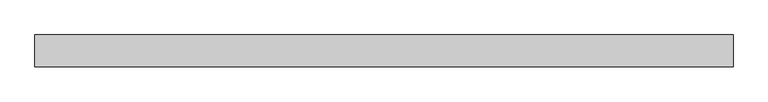
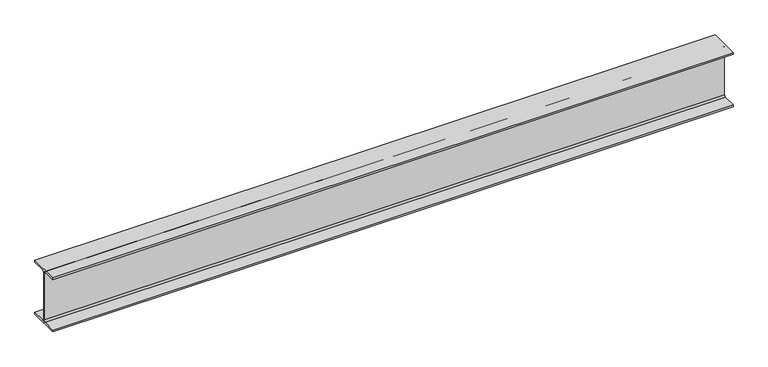
"""IFC4 building model written with IfcOpenShell, lengths in millimetres: beam geometry, Old_Steel Beam_H-KSD3502 : H_SB_ASB_H-250×125x6x9."""

from ifc_helpers import new_model, si_unit, point, frame, frame_2d, origin, place, context, project, spatial, polyline, circle_curve, trimmed, segment, composite_curve, outline, extrude, source, transform, mapped, element, save


def beam_e590c642(model_context):
    return source(origin(), model_context, "Body", "SweptSolid", [
        extrude(outline(composite_curve([segment(polyline([(82.5, -141.5), (82.5, -151.7), (-82.5, -151.7), (-82.5, -141.5), (-11.9, -141.5)]), True, "CONTINUOUS"), segment(trimmed(circle_curve(frame_2d((-11.9, -132.6)), 8.9), [point((-11.9, -141.5))], [point((-3.0, -132.6))], True, "CARTESIAN"), True, "CONTINUOUS"), segment(polyline([(-3.0, -132.6), (-3.0, 132.6)]), True, "CONTINUOUS"), segment(trimmed(circle_curve(frame_2d((-11.9, 132.6)), 8.9), [point((-3.0, 132.6))], [point((-11.9, 141.5))], True, "CARTESIAN"), True, "CONTINUOUS"), segment(polyline([(-11.9, 141.5), (-82.5, 141.5), (-82.5, 151.7), (82.5, 151.7), (82.5, 141.5), (11.9, 141.5)]), True, "CONTINUOUS"), segment(trimmed(circle_curve(frame_2d((11.9, 132.6)), 8.9), [point((11.9, 141.5))], [point((3.0, 132.6))], True, "CARTESIAN"), True, "CONTINUOUS"), segment(polyline([(3.0, 132.6), (3.0, -132.6)]), True, "CONTINUOUS"), segment(trimmed(circle_curve(frame_2d((11.9, -132.6)), 8.9), [point((3.0, -132.6))], [point((11.9, -141.5))], True, "CARTESIAN"), True, "CONTINUOUS"), segment(polyline([(11.9, -141.5), (82.5, -141.5)]), True, "CONTINUOUS")], self_intersect=False)), frame((-1718.3833333, 0.0, 0.0), z_axis=(1.0, 0.0, 0.0), x_axis=(0.0, 1.0, 0.0)), (0.0, 0.0, 1.0), 3623.1833333),
    ])


if __name__ == "__main__":
    model = new_model("IFC4")
    model_context = context("Model", 3, world=origin())
    ifc_project = project(units=[si_unit("LENGTHUNIT", "METRE", prefix="MILLI")], contexts=[model_context])
    site = spatial("IfcSite", under=ifc_project)
    building = spatial("IfcBuilding", under=site)
    placement = place(None, origin())
    beam_shape = beam_e590c642(model_context)
    element("IfcBeam", 1, ObjectType="Old_Steel Beam_H-KSD3502 : H_SB_ASB_H-250×125x6x9", at=placement, inside=building, context=model_context, shape_type="MappedRepresentation", body=[
        mapped(beam_shape, transform((0.0, 0.0, 0.0), x_axis=(1.0, 0.0, 0.0), y_axis=(0.0, 1.0, 0.0), z_axis=(0.0, 0.0, 1.0))),
    ])
    save(model, "model.ifc")

# Revit data of these elements
# Type "Old_Steel Beam_H-KSD3502 : H_SB_ASB_H-250×125x6x9"
#   Width = 12.5 cm
#   Web Thickness = 0.6 cm
#   Web Fillet = 1.2 cm
#   Warping Constant = 42539.8 cm⁶
#   Torsional Moment of Inertia = 7.8102 cm⁴
#   Torsional Modulus = 1.0 cm³
#   Section Area = 37.66 cm²
#   Plastic Modulus weak axis = 73.1 cm³
#   Plastic Modulus strong axis = 366.0 cm³
#   Perimeter = 0.97 m²/m
#   Nominal Weight = 29.60 kgf/m
#   Moment of Inertia weak axis = 294.00 cm⁴
#   Moment of Inertia strong axis = 4050.00 cm⁴
#   Height = 25.0 cm
#   Flange Thickness = 0.9 cm
#   Elastic Modulus weak axis = 47.0 cm³
#   Elastic Modulus strong axis = 324.0 cm³
#   Centroid Vertical = 12.5 cm
#   Centroid Horizontal = 6.25 cm
#   Length [instance default] = 1.5240 m
#   Structural Material [instance default] = Steel, 45-345
#   Assembly Code = ""
# Element 1 (IfcBeam, "Old_Steel Beam_H-KSD3502 : H_SB_ASB_H-250×125x6x9")
#   Structural Material = none
# Materials
#   "Steel, 45-345": class "Metal", colour RGB 189 187 185, transparency 0, Description = "Steel 345 MPa", Cost = 0
